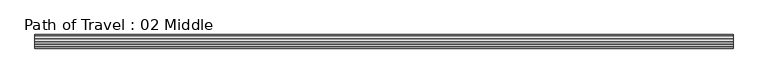
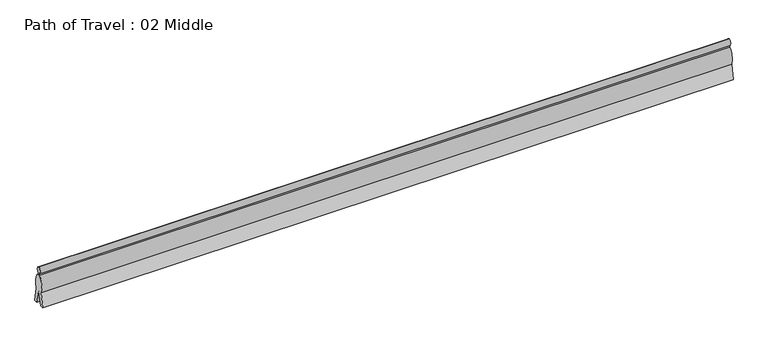
"""IFC4 building model written with IfcOpenShell, lengths in millimetres: proxy geometry, Path of Travel : 02 Middle."""

from ifc_helpers import new_model, si_unit, point, frame, origin, place, context, project, spatial, ellipse_curve, trimmed, source, transform, mapped, element, save
from ifc_brep_helpers import plane_surface, extruded_surface, advanced_brep


def path_of_travel_02_middle_a6952bb6(model_context):
    return source(origin(), model_context, "Body", "AdvancedBrep", [
        advanced_brep(
        [(227.5554837, 0.0, 1727.2), (227.5554837, 42.9018657, 1436.6534209), (227.5554837, 42.9018657, 1363.4763406), (227.5554837, 184.1186263, 643.4144547), (227.5554837, 297.5699544, 0.0), (227.5554837, 145.6574193, 0.0), (227.5554837, 0.0, 584.2), (227.5554837, -145.6574193, 0.0), (227.5554837, -297.5699544, 0.0), (227.5554837, -184.1186263, 643.4144547), (227.5554837, -42.9018657, 1363.4763406), (227.5554837, -42.9018657, 1436.6534209), (30707.5554837, 0.0, 1727.2), (30707.5554837, -42.9018657, 1436.6534209), (30707.5554837, -42.9018657, 1363.4763406), (30707.5554837, -184.1186263, 643.4144547), (30707.5554837, -297.5699544, 0.0), (30707.5554837, -145.6574193, 0.0), (30707.5554837, 0.0, 584.2), (30707.5554837, 145.6574193, 0.0), (30707.5554837, 297.5699544, 0.0), (30707.5554837, 184.1186263, 643.4144547), (30707.5554837, 42.9018657, 1363.4763406), (30707.5554837, 42.9018657, 1436.6534209)],
        [
            (0, 1, ellipse_curve(frame((227.5554837, 0.0, 1574.8), z_axis=(-1.0, 0.0, 0.0), x_axis=(0.0, 0.0, 1.0)), 152.4, 101.6)),
            (1, 2),
            (2, 3, ellipse_curve(frame((227.5554837, 0.0, 914.4), z_axis=(-1.0, 0.0, 0.0), x_axis=(0.0, 0.0, -1.0)), 457.2, 228.6)),
            (3, 4),
            (4, 5),
            (5, 6),
            (6, 7),
            (7, 8),
            (8, 9),
            (9, 10, ellipse_curve(frame((227.5554837, 0.0, 914.4), z_axis=(-1.0, 0.0, 0.0), x_axis=(0.0, 0.0, -1.0)), 457.2, 228.6)),
            (10, 11),
            (11, 0, ellipse_curve(frame((227.5554837, 0.0, 1574.8), z_axis=(-1.0, 0.0, 0.0), x_axis=(0.0, 0.0, 1.0)), 152.4, 101.6)),
            (12, 13, ellipse_curve(frame((30707.5554837, 0.0, 1574.8), z_axis=(1.0, 0.0, 0.0), x_axis=(0.0, 0.0, 1.0)), 152.4, 101.6)),
            (13, 14),
            (14, 15, ellipse_curve(frame((30707.5554837, 0.0, 914.4), z_axis=(1.0, 0.0, 0.0), x_axis=(0.0, 0.0, -1.0)), 457.2, 228.6)),
            (15, 16),
            (16, 17),
            (17, 18),
            (18, 19),
            (19, 20),
            (20, 21),
            (21, 22, ellipse_curve(frame((30707.5554837, 0.0, 914.4), z_axis=(1.0, 0.0, 0.0), x_axis=(0.0, 0.0, -1.0)), 457.2, 228.6)),
            (22, 23),
            (23, 12, ellipse_curve(frame((30707.5554837, 0.0, 1574.8), z_axis=(1.0, 0.0, 0.0), x_axis=(0.0, 0.0, 1.0)), 152.4, 101.6)),
            (0, 12),
            (23, 1),
            (22, 2),
            (21, 3),
            (20, 4),
            (19, 5),
            (18, 6),
            (17, 7),
            (16, 8),
            (15, 9),
            (14, 10),
            (13, 11),
        ],
        [
            plane_surface(frame((227.5554837, 0.0, 0.0), z_axis=(-1.0, 0.0, 0.0), x_axis=(0.0, 0.0, 1.0))),
            plane_surface(frame((30707.5554837, 0.0, 0.0), z_axis=(1.0, 0.0, 0.0), x_axis=(0.0, 0.0, 1.0))),
            extruded_surface(trimmed(ellipse_curve(frame((30707.5554837, 0.0, 1574.8), z_axis=(-1.0, 0.0, 0.0), x_axis=(0.0, 0.0, 1.0)), 152.4, 101.6), [point((30707.5554837, 0.0, 1727.2))], [point((30707.5554837, 42.9018657, 1436.6534209))], True, "CARTESIAN"), (-30480.0, 0.0, 0.0), 30480.0),
            plane_surface(frame((227.5554837, 42.9018657, 1436.6534209), z_axis=(0.0, 1.0, 0.0), x_axis=(1.0, 0.0, 0.0))),
            extruded_surface(trimmed(ellipse_curve(frame((30707.5554837, 0.0, 914.4), z_axis=(-1.0, 0.0, 0.0), x_axis=(0.0, 0.0, -1.0)), 457.2, 228.6), [point((30707.5554837, 42.9018657, 1363.4763406))], [point((30707.5554837, 184.1186263, 643.4144547))], True, "CARTESIAN"), (-30480.0, 0.0, 0.0), 30480.0),
            plane_surface(frame((227.5554837, 184.1186263, 643.4144547), z_axis=(0.0, 0.9848077530122078, 0.17364817766693205), x_axis=(1.0, 0.0, 0.0))),
            plane_surface(frame((227.5554837, 297.5699544, 0.0), z_axis=(0.0, 0.0, -1.0), x_axis=(1.0, 0.0, 0.0))),
            plane_surface(frame((227.5554837, 145.6574193, 0.0), z_axis=(0.0, -0.9702957262760199, -0.2419218955995739), x_axis=(1.0, 0.0, 0.0))),
            plane_surface(frame((227.5554837, 0.0, 584.2), z_axis=(0.0, 0.9702957262759961, -0.24192189559966923), x_axis=(1.0, 0.0, 0.0))),
            plane_surface(frame((227.5554837, -145.6574193, 0.0), z_axis=(0.0, 0.0, -1.0), x_axis=(1.0, 0.0, 0.0))),
            plane_surface(frame((227.5554837, -297.5699544, 0.0), z_axis=(0.0, -0.984807753012208, 0.17364817766693066), x_axis=(1.0, 0.0, 0.0))),
            extruded_surface(trimmed(ellipse_curve(frame((30707.5554837, 0.0, 914.4), z_axis=(-1.0, 0.0, 0.0), x_axis=(0.0, 0.0, -1.0)), 457.2, 228.6), [point((30707.5554837, -184.1186263, 643.4144547))], [point((30707.5554837, -42.9018657, 1363.4763406))], True, "CARTESIAN"), (-30480.0, 0.0, 0.0), 30480.0),
            plane_surface(frame((227.5554837, -42.9018657, 1363.4763406), z_axis=(0.0, -1.0, 0.0), x_axis=(1.0, 0.0, 0.0))),
            extruded_surface(trimmed(ellipse_curve(frame((30707.5554837, 0.0, 1574.8), z_axis=(-1.0, 0.0, 0.0), x_axis=(0.0, 0.0, 1.0)), 152.4, 101.6), [point((30707.5554837, -42.9018657, 1436.6534209))], [point((30707.5554837, 0.0, 1727.2))], True, "CARTESIAN"), (-30480.0, 0.0, 0.0), 30480.0),
        ],
        [
            (0, [[1, 2, 3, 4, 5, 6, 7, 8, 9, 10, 11, 12]]),
            (1, [[13, 14, 15, 16, 17, 18, 19, 20, 21, 22, 23, 24]]),
            (2, [[-1, 25, -24, 26]]),
            (3, [[-2, -26, -23, 27]]),
            (4, [[-3, -27, -22, 28]]),
            (5, [[-4, -28, -21, 29]]),
            (6, [[-5, -29, -20, 30]]),
            (7, [[-6, -30, -19, 31]]),
            (8, [[-7, -31, -18, 32]]),
            (9, [[-8, -32, -17, 33]]),
            (10, [[-9, -33, -16, 34]]),
            (11, [[-10, -34, -15, 35]]),
            (12, [[-11, -35, -14, 36]]),
            (13, [[-12, -36, -13, -25]]),
        ],
    ),
    ])


if __name__ == "__main__":
    model = new_model("IFC4")
    model_context = context("Model", 3, world=origin())
    ifc_project = project(units=[si_unit("LENGTHUNIT", "METRE", prefix="MILLI")], contexts=[model_context])
    site = spatial("IfcSite", under=ifc_project)
    building = spatial("IfcBuilding", under=site)
    placement = place(None, origin())
    path_of_travel_02_middle_shape = path_of_travel_02_middle_a6952bb6(model_context)
    element("IfcBuildingElementProxy", 1, Name="Path of Travel : 02 Middle", ObjectType="Path of Travel : 02 Middle", at=placement, inside=building, context=model_context, shape_type="MappedRepresentation", body=[
        mapped(path_of_travel_02_middle_shape, transform((0.0, 0.0, 0.0), x_axis=(1.0, 0.0, 0.0), y_axis=(0.0, 1.0, 0.0), z_axis=(0.0, 0.0, 1.0))),
    ])
    save(model, "model.ifc")

# Revit data of these elements
# Type "Path of Travel : 02 Middle"
#   Path of Egress [instance default] = 4' - 0"
#   built-in parameter 1001306 [instance default] = 4 (stored number, unit not read)
#   Dot at Start = no
#   Arrow in Middle = yes
#   Arrow at End = no
#   Egress Path = none
# Element 1 (IfcBuildingElementProxy, "Path of Travel : 02 Middle")
#   Path of Egress = 100' - 0"
#   built-in parameter 1001306 = 100 (stored number, unit not read)
#   Materials on its faces: "Egress Path Solid"
# Materials
#   "Egress Path Solid": class "Unassigned", colour RGB 255 128 64, transparency 0.75, Comments = "Rendering appearance not upgraded "
